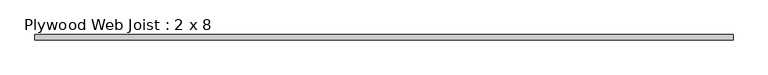
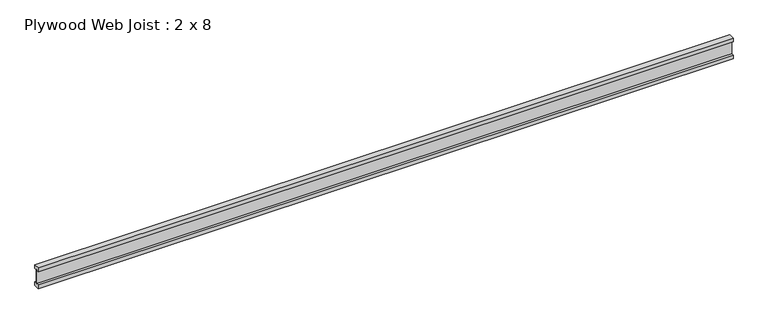
"""IFC4 building model written with IfcOpenShell, lengths in millimetres: beam geometry, Plywood Web Joist : 2 x 8."""

import ifcopenshell
import ifcopenshell.guid

model = None  # the IFC model being written
_history = None  # IfcOwnerHistory: only IFC2X3 demands one
_inside = {}  # id of a spatial element -> (the spatial element, [elements in it])
_under = {}  # id of a project, library or spatial element -> (it, [spatial elements below it])
_declared = {}  # id of a project -> (the project, [libraries it declares])
_typed = {}  # id of a type object -> (the type object, [elements of that type])
_made_of = {}  # id of a material, layer set ... -> (it, [elements and type objects made of it])


def new_model(schema):
    """Start an empty IFC model of exactly this schema.

    Asked for "IFC4X3", IfcOpenShell would pick the latest addendum, in which some entities
    have other attributes; the version numbers below select the first issue.
    IFC2X3 requires an IfcOwnerHistory on every rooted entity: one is made here for all.
    """
    global model, _history
    if schema == "IFC4X3":
        model = ifcopenshell.file(schema_version=(4, 3, 0, 0))
    else:
        model = ifcopenshell.file(schema=schema)
    _inside.clear()
    _under.clear()
    _declared.clear()
    _typed.clear()
    _made_of.clear()
    _history = None
    if model.schema == "IFC2X3":
        org = make("IfcOrganization", Name="unknown")
        user = make(
            "IfcPersonAndOrganization",
            ThePerson=make("IfcPerson", FamilyName="unknown"),
            TheOrganization=org,
        )
        app = make(
            "IfcApplication",
            ApplicationDeveloper=org,
            Version="unknown",
            ApplicationFullName="unknown",
            ApplicationIdentifier="unknown",
        )
        _history = make(
            "IfcOwnerHistory",
            OwningUser=user,
            OwningApplication=app,
            ChangeAction="ADDED",
            CreationDate=0,
        )
    return model


def make(cls, **values):
    """One entity of the class cls with the attributes given. An attribute that is None is left unset."""
    return model.create_entity(
        cls, **{name: value for name, value in values.items() if value is not None}
    )


def rooted(cls, **values):
    """An entity with a GlobalId (a new one), such as an element, a storey or a relation."""
    return make(cls, GlobalId=ifcopenshell.guid.new(), OwnerHistory=_history, **values)


def si_unit(unit_type, name, prefix=None):
    """IfcSIUnit, for example si_unit("LENGTHUNIT", "METRE", prefix="MILLI")."""
    return make("IfcSIUnit", UnitType=unit_type, Prefix=prefix, Name=name)


def assignment(units):
    """IfcUnitAssignment: the units of a project."""
    return None if units is None else make("IfcUnitAssignment", Units=units)


def point(xyz):
    """IfcCartesianPoint."""
    return None if xyz is None else make("IfcCartesianPoint", Coordinates=xyz)


def direction(xyz):
    """IfcDirection."""
    return None if xyz is None else make("IfcDirection", DirectionRatios=xyz)


def frame(location, z_axis=None, x_axis=None):
    """IfcAxis2Placement3D, a coordinate frame: its origin and axes. An axis left out is left unset."""
    return make(
        "IfcAxis2Placement3D",
        Location=point(location),
        Axis=direction(z_axis),
        RefDirection=direction(x_axis),
    )


def origin():
    """The frame at (0, 0, 0) with its axes left unset."""
    return frame((0.0, 0.0, 0.0))


def place(relative_to, where):
    """IfcLocalPlacement: puts the frame where relative to a parent placement (None: the world)."""
    return make(
        "IfcLocalPlacement", PlacementRelTo=relative_to, RelativePlacement=where
    )


def context(
    kind, dimensions, precision=None, world=None, true_north=None, identifier=None
):
    """IfcGeometricRepresentationContext, for example the 3D "Model" context."""
    return make(
        "IfcGeometricRepresentationContext",
        ContextIdentifier=identifier,
        ContextType=kind,
        CoordinateSpaceDimension=dimensions,
        Precision=precision,
        WorldCoordinateSystem=world,
        TrueNorth=true_north,
    )


def project(units=None, contexts=None):
    """IfcProject with its units and contexts."""
    return rooted(
        "IfcProject",
        Name="project",
        RepresentationContexts=contexts,
        UnitsInContext=assignment(units),
    )


def spatial(cls, under=None, at=None, **own):
    """A site, building, storey or space (cls), placed at a placement, below another one or the project."""
    s = rooted(cls, ObjectPlacement=at, **own)
    if under is not None:
        _under.setdefault(under.id(), (under, []))[1].append(s)
    return s


def polyline(points):
    """IfcPolyline through the points."""
    return make("IfcPolyline", Points=[point(p) for p in points])


def outline(outer, holes=None, kind="AREA"):
    """IfcArbitraryClosedProfileDef: a profile drawn as a closed curve; with holes, ...WithVoids."""
    if holes is None:
        return make("IfcArbitraryClosedProfileDef", ProfileType=kind, OuterCurve=outer)
    return make(
        "IfcArbitraryProfileDefWithVoids",
        ProfileType=kind,
        OuterCurve=outer,
        InnerCurves=holes,
    )


def extrude(swept, where, along, depth):
    """IfcExtrudedAreaSolid: the profile swept, set in the frame where, extruded along a direction by depth."""
    return make(
        "IfcExtrudedAreaSolid",
        SweptArea=swept,
        Position=where,
        ExtrudedDirection=direction(along),
        Depth=depth,
    )


def shape(context_of_items, identifier, shape_type, items):
    """IfcShapeRepresentation: the items that make up one representation, for example the "Body"."""
    return make(
        "IfcShapeRepresentation",
        ContextOfItems=context_of_items,
        RepresentationIdentifier=identifier,
        RepresentationType=shape_type,
        Items=items,
    )


def source(mapping_origin, context_of_items, identifier, shape_type, items):
    """IfcRepresentationMap: a shape defined once, which mapped items show again and again."""
    return make(
        "IfcRepresentationMap",
        MappingOrigin=mapping_origin,
        MappedRepresentation=shape(context_of_items, identifier, shape_type, items),
    )


def transform(
    local_origin,
    x_axis=None,
    y_axis=None,
    z_axis=None,
    scale=None,
    scale2=None,
    scale3=None,
    uniform=True,
):
    """IfcCartesianTransformationOperator3D, or its non-uniform kind. x_axis, y_axis, z_axis: its Axis1, 2, 3."""
    if uniform:
        return make(
            "IfcCartesianTransformationOperator3D",
            Axis1=direction(x_axis),
            Axis2=direction(y_axis),
            LocalOrigin=point(local_origin),
            Scale=scale,
            Axis3=direction(z_axis),
        )
    return make(
        "IfcCartesianTransformationOperator3DnonUniform",
        Axis1=direction(x_axis),
        Axis2=direction(y_axis),
        LocalOrigin=point(local_origin),
        Scale=scale,
        Axis3=direction(z_axis),
        Scale2=scale2,
        Scale3=scale3,
    )


def mapped(mapping_source, mapping_target):
    """IfcMappedItem: shows the shape of a source again, moved by a transform."""
    return make(
        "IfcMappedItem", MappingSource=mapping_source, MappingTarget=mapping_target
    )


def made_of(thing, what):
    """Note that an element or type object is made of a material, layer set ...; save() writes the relation."""
    if what is not None:
        _made_of.setdefault(what.id(), (what, []))[1].append(thing)
    return thing


def element(
    cls,
    number,
    at=None,
    inside=None,
    cuts=None,
    type_object=None,
    material=None,
    context=None,
    identifier="Body",
    shape_type=None,
    held_by="IfcProductDefinitionShape",
    body=None,
    shapes=None,
    **own,
):
    """One element of the class cls, such as IfcWall. Its Tag is "e" and its number.

    at: its placement. inside: the storey or other place that contains it. cuts: it is an
    opening in that element (IfcRelVoidsElement). A single representation is given by context,
    identifier, shape_type and body (its items); several are given by shapes. held_by: the class
    of the entity that holds the representations. save() writes the other relations.
    """
    e = rooted(cls, Tag="e%d" % number, ObjectPlacement=at, **own)
    if body is not None:
        shapes = [shape(context, identifier, shape_type, body)]
    if shapes is not None:
        e.Representation = make(held_by, Representations=shapes)
    if inside is not None:
        _inside.setdefault(inside.id(), (inside, []))[1].append(e)
    if cuts is not None:
        rooted(
            "IfcRelVoidsElement", RelatingBuildingElement=cuts, RelatedOpeningElement=e
        )
    if type_object is not None:
        _typed.setdefault(type_object.id(), (type_object, []))[1].append(e)
    return made_of(e, material)


def aggregate(whole, parts):
    """IfcRelAggregates: a whole, such as a stair, and the parts it consists of."""
    return rooted("IfcRelAggregates", RelatingObject=whole, RelatedObjects=parts)


def save(model, path):
    """Write the relations noted so far, then the file.

    IfcRelAggregates (storeys below a building ...), IfcRelContainedInSpatialStructure (elements
    in a storey), IfcRelDefinesByType, IfcRelAssociatesMaterial and IfcRelDeclares: one each for
    every whole, place, type object, material and project.
    """
    for whole, parts in _under.values():
        aggregate(whole, parts)
    for where, things in _inside.values():
        rooted(
            "IfcRelContainedInSpatialStructure",
            RelatedElements=things,
            RelatingStructure=where,
        )
    for kind, things in _typed.values():
        rooted("IfcRelDefinesByType", RelatedObjects=things, RelatingType=kind)
    for what, things in _made_of.values():
        rooted("IfcRelAssociatesMaterial", RelatedObjects=things, RelatingMaterial=what)
    for by, libraries in _declared.values():
        rooted("IfcRelDeclares", RelatingContext=by, RelatedDefinitions=libraries)
    model.write(path)


def plywood_web_joist_2_x_8_156d774c(model_context):
    return source(origin(), model_context, "Body", "SweptSolid", [
        extrude(outline(polyline([(-25.4, 101.6), (25.4, 101.6), (25.4, 63.5), (4.7625, 63.5), (4.7625, 69.85), (-4.7625, 69.85), (-4.7625, 63.5), (-25.4, 63.5), (-25.4, 101.6)])), frame((-3195.5616975, 0.0, 0.0), z_axis=(1.0, 0.0, 0.0), x_axis=(0.0, 1.0, 0.0)), (0.0, 0.0, 1.0), 6391.1233951),
        extrude(outline(polyline([(25.4, -63.5), (25.4, -101.6), (-25.4, -101.6), (-25.4, -63.5), (-4.7625, -63.5), (-4.7625, -69.1160374), (4.7625, -69.1160374), (4.7625, -63.5), (25.4, -63.5)])), frame((-3195.5616975, 0.0, 0.0), z_axis=(1.0, 0.0, 0.0), x_axis=(0.0, 1.0, 0.0)), (0.0, 0.0, 1.0), 6391.1233951),
        extrude(outline(polyline([(3195.5616975, 4.7625), (3195.5616975, -4.7625), (-3195.5616975, -4.7625), (-3195.5616975, 4.7625), (3195.5616975, 4.7625)])), frame((0.0, 0.0, -69.1160374), z_axis=(0.0, 0.0, 1.0), x_axis=(1.0, 0.0, 0.0)), (0.0, 0.0, 1.0), 138.9660374),
    ])


if __name__ == "__main__":
    model = new_model("IFC4")
    model_context = context("Model", 3, world=origin())
    ifc_project = project(units=[si_unit("LENGTHUNIT", "METRE", prefix="MILLI")], contexts=[model_context])
    site = spatial("IfcSite", under=ifc_project)
    building = spatial("IfcBuilding", under=site)
    placement = place(None, origin())
    plywood_web_joist_2_x_8_shape = plywood_web_joist_2_x_8_156d774c(model_context)
    element("IfcBeam", 1, ObjectType="Plywood Web Joist : 2 x 8", at=placement, inside=building, context=model_context, shape_type="MappedRepresentation", body=[
        mapped(plywood_web_joist_2_x_8_shape, transform((0.0, 0.0, 0.0), x_axis=(1.0, 0.0, 0.0), y_axis=(0.0, 1.0, 0.0), z_axis=(0.0, 0.0, 1.0))),
    ])
    save(model, "model.ifc")

# Revit data of these elements
# Type "Plywood Web Joist : 2 x 8"
#   Assembly Code = "B10"
#   Length [instance default] = 5' - 0"
#   b = 0' - 2"
#   d = 0' - 8"
#   Structural Material [instance default] = Softwood, Lumber
# Element 1 (IfcBeam, "Plywood Web Joist : 2 x 8")
#   Materials on its faces: "Softwood, Lumber"
# Materials
#   "Softwood, Lumber": class "Wood", colour RGB 144 113 62, transparency 0, Description = "Pinus Echinata", Cost = 0
